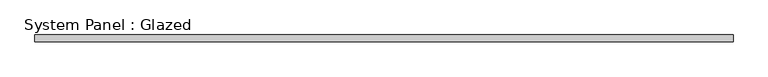
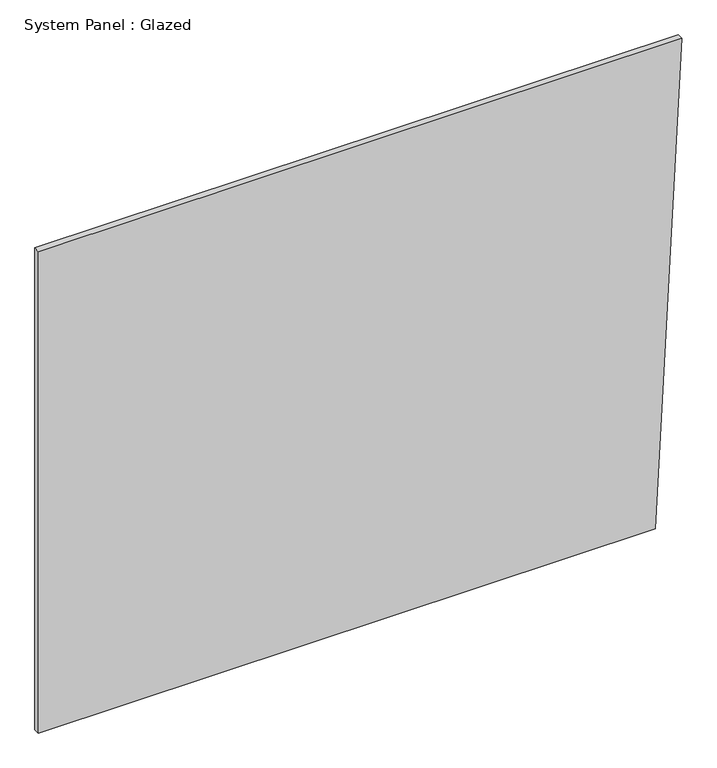
"""IFC4 building model written with IfcOpenShell, lengths in millimetres: plate geometry, System Panel : Glazed."""

import ifcopenshell
import ifcopenshell.guid

model = None  # the IFC model being written
_history = None  # IfcOwnerHistory: only IFC2X3 demands one
_inside = {}  # id of a spatial element -> (the spatial element, [elements in it])
_under = {}  # id of a project, library or spatial element -> (it, [spatial elements below it])
_declared = {}  # id of a project -> (the project, [libraries it declares])
_typed = {}  # id of a type object -> (the type object, [elements of that type])
_made_of = {}  # id of a material, layer set ... -> (it, [elements and type objects made of it])


def new_model(schema):
    """Start an empty IFC model of exactly this schema.

    Asked for "IFC4X3", IfcOpenShell would pick the latest addendum, in which some entities
    have other attributes; the version numbers below select the first issue.
    IFC2X3 requires an IfcOwnerHistory on every rooted entity: one is made here for all.
    """
    global model, _history
    if schema == "IFC4X3":
        model = ifcopenshell.file(schema_version=(4, 3, 0, 0))
    else:
        model = ifcopenshell.file(schema=schema)
    _inside.clear()
    _under.clear()
    _declared.clear()
    _typed.clear()
    _made_of.clear()
    _history = None
    if model.schema == "IFC2X3":
        org = make("IfcOrganization", Name="unknown")
        user = make(
            "IfcPersonAndOrganization",
            ThePerson=make("IfcPerson", FamilyName="unknown"),
            TheOrganization=org,
        )
        app = make(
            "IfcApplication",
            ApplicationDeveloper=org,
            Version="unknown",
            ApplicationFullName="unknown",
            ApplicationIdentifier="unknown",
        )
        _history = make(
            "IfcOwnerHistory",
            OwningUser=user,
            OwningApplication=app,
            ChangeAction="ADDED",
            CreationDate=0,
        )
    return model


def make(cls, **values):
    """One entity of the class cls with the attributes given. An attribute that is None is left unset."""
    return model.create_entity(
        cls, **{name: value for name, value in values.items() if value is not None}
    )


def rooted(cls, **values):
    """An entity with a GlobalId (a new one), such as an element, a storey or a relation."""
    return make(cls, GlobalId=ifcopenshell.guid.new(), OwnerHistory=_history, **values)


def si_unit(unit_type, name, prefix=None):
    """IfcSIUnit, for example si_unit("LENGTHUNIT", "METRE", prefix="MILLI")."""
    return make("IfcSIUnit", UnitType=unit_type, Prefix=prefix, Name=name)


def assignment(units):
    """IfcUnitAssignment: the units of a project."""
    return None if units is None else make("IfcUnitAssignment", Units=units)


def point(xyz):
    """IfcCartesianPoint."""
    return None if xyz is None else make("IfcCartesianPoint", Coordinates=xyz)


def direction(xyz):
    """IfcDirection."""
    return None if xyz is None else make("IfcDirection", DirectionRatios=xyz)


def frame(location, z_axis=None, x_axis=None):
    """IfcAxis2Placement3D, a coordinate frame: its origin and axes. An axis left out is left unset."""
    return make(
        "IfcAxis2Placement3D",
        Location=point(location),
        Axis=direction(z_axis),
        RefDirection=direction(x_axis),
    )


def origin():
    """The frame at (0, 0, 0) with its axes left unset."""
    return frame((0.0, 0.0, 0.0))


def place(relative_to, where):
    """IfcLocalPlacement: puts the frame where relative to a parent placement (None: the world)."""
    return make(
        "IfcLocalPlacement", PlacementRelTo=relative_to, RelativePlacement=where
    )


def context(
    kind, dimensions, precision=None, world=None, true_north=None, identifier=None
):
    """IfcGeometricRepresentationContext, for example the 3D "Model" context."""
    return make(
        "IfcGeometricRepresentationContext",
        ContextIdentifier=identifier,
        ContextType=kind,
        CoordinateSpaceDimension=dimensions,
        Precision=precision,
        WorldCoordinateSystem=world,
        TrueNorth=true_north,
    )


def project(units=None, contexts=None):
    """IfcProject with its units and contexts."""
    return rooted(
        "IfcProject",
        Name="project",
        RepresentationContexts=contexts,
        UnitsInContext=assignment(units),
    )


def spatial(cls, under=None, at=None, **own):
    """A site, building, storey or space (cls), placed at a placement, below another one or the project."""
    s = rooted(cls, ObjectPlacement=at, **own)
    if under is not None:
        _under.setdefault(under.id(), (under, []))[1].append(s)
    return s


def polyline(points):
    """IfcPolyline through the points."""
    return make("IfcPolyline", Points=[point(p) for p in points])


def outline(outer, holes=None, kind="AREA"):
    """IfcArbitraryClosedProfileDef: a profile drawn as a closed curve; with holes, ...WithVoids."""
    if holes is None:
        return make("IfcArbitraryClosedProfileDef", ProfileType=kind, OuterCurve=outer)
    return make(
        "IfcArbitraryProfileDefWithVoids",
        ProfileType=kind,
        OuterCurve=outer,
        InnerCurves=holes,
    )


def extrude(swept, where, along, depth):
    """IfcExtrudedAreaSolid: the profile swept, set in the frame where, extruded along a direction by depth."""
    return make(
        "IfcExtrudedAreaSolid",
        SweptArea=swept,
        Position=where,
        ExtrudedDirection=direction(along),
        Depth=depth,
    )


def shape(context_of_items, identifier, shape_type, items):
    """IfcShapeRepresentation: the items that make up one representation, for example the "Body"."""
    return make(
        "IfcShapeRepresentation",
        ContextOfItems=context_of_items,
        RepresentationIdentifier=identifier,
        RepresentationType=shape_type,
        Items=items,
    )


def source(mapping_origin, context_of_items, identifier, shape_type, items):
    """IfcRepresentationMap: a shape defined once, which mapped items show again and again."""
    return make(
        "IfcRepresentationMap",
        MappingOrigin=mapping_origin,
        MappedRepresentation=shape(context_of_items, identifier, shape_type, items),
    )


def transform(
    local_origin,
    x_axis=None,
    y_axis=None,
    z_axis=None,
    scale=None,
    scale2=None,
    scale3=None,
    uniform=True,
):
    """IfcCartesianTransformationOperator3D, or its non-uniform kind. x_axis, y_axis, z_axis: its Axis1, 2, 3."""
    if uniform:
        return make(
            "IfcCartesianTransformationOperator3D",
            Axis1=direction(x_axis),
            Axis2=direction(y_axis),
            LocalOrigin=point(local_origin),
            Scale=scale,
            Axis3=direction(z_axis),
        )
    return make(
        "IfcCartesianTransformationOperator3DnonUniform",
        Axis1=direction(x_axis),
        Axis2=direction(y_axis),
        LocalOrigin=point(local_origin),
        Scale=scale,
        Axis3=direction(z_axis),
        Scale2=scale2,
        Scale3=scale3,
    )


def mapped(mapping_source, mapping_target):
    """IfcMappedItem: shows the shape of a source again, moved by a transform."""
    return make(
        "IfcMappedItem", MappingSource=mapping_source, MappingTarget=mapping_target
    )


def made_of(thing, what):
    """Note that an element or type object is made of a material, layer set ...; save() writes the relation."""
    if what is not None:
        _made_of.setdefault(what.id(), (what, []))[1].append(thing)
    return thing


def element(
    cls,
    number,
    at=None,
    inside=None,
    cuts=None,
    type_object=None,
    material=None,
    context=None,
    identifier="Body",
    shape_type=None,
    held_by="IfcProductDefinitionShape",
    body=None,
    shapes=None,
    **own,
):
    """One element of the class cls, such as IfcWall. Its Tag is "e" and its number.

    at: its placement. inside: the storey or other place that contains it. cuts: it is an
    opening in that element (IfcRelVoidsElement). A single representation is given by context,
    identifier, shape_type and body (its items); several are given by shapes. held_by: the class
    of the entity that holds the representations. save() writes the other relations.
    """
    e = rooted(cls, Tag="e%d" % number, ObjectPlacement=at, **own)
    if body is not None:
        shapes = [shape(context, identifier, shape_type, body)]
    if shapes is not None:
        e.Representation = make(held_by, Representations=shapes)
    if inside is not None:
        _inside.setdefault(inside.id(), (inside, []))[1].append(e)
    if cuts is not None:
        rooted(
            "IfcRelVoidsElement", RelatingBuildingElement=cuts, RelatedOpeningElement=e
        )
    if type_object is not None:
        _typed.setdefault(type_object.id(), (type_object, []))[1].append(e)
    return made_of(e, material)


def aggregate(whole, parts):
    """IfcRelAggregates: a whole, such as a stair, and the parts it consists of."""
    return rooted("IfcRelAggregates", RelatingObject=whole, RelatedObjects=parts)


def save(model, path):
    """Write the relations noted so far, then the file.

    IfcRelAggregates (storeys below a building ...), IfcRelContainedInSpatialStructure (elements
    in a storey), IfcRelDefinesByType, IfcRelAssociatesMaterial and IfcRelDeclares: one each for
    every whole, place, type object, material and project.
    """
    for whole, parts in _under.values():
        aggregate(whole, parts)
    for where, things in _inside.values():
        rooted(
            "IfcRelContainedInSpatialStructure",
            RelatedElements=things,
            RelatingStructure=where,
        )
    for kind, things in _typed.values():
        rooted("IfcRelDefinesByType", RelatedObjects=things, RelatingType=kind)
    for what, things in _made_of.values():
        rooted("IfcRelAssociatesMaterial", RelatedObjects=things, RelatingMaterial=what)
    for by, libraries in _declared.values():
        rooted("IfcRelDeclares", RelatingContext=by, RelatedDefinitions=libraries)
    model.write(path)


def system_panel_glazed_f6a0a944(model_context):
    return source(origin(), model_context, "Body", "SweptSolid", [
        extrude(outline(polyline([(0.0, -1317.8741594), (0.0, 1208.7338763), (2085.3785982, 1317.8741594), (2085.3785982, -1317.8741594), (0.0, -1317.8741594)])), frame((0.0, -44.45, 0.0), z_axis=(0.0, 1.0, 0.0), x_axis=(0.0, 0.0, 1.0)), (0.0, 0.0, 1.0), 25.4),
    ])


if __name__ == "__main__":
    model = new_model("IFC4")
    model_context = context("Model", 3, world=origin())
    ifc_project = project(units=[si_unit("LENGTHUNIT", "METRE", prefix="MILLI")], contexts=[model_context])
    site = spatial("IfcSite", under=ifc_project)
    building = spatial("IfcBuilding", under=site)
    placement = place(None, origin())
    system_panel_glazed_shape = system_panel_glazed_f6a0a944(model_context)
    element("IfcPlate", 1, ObjectType="System Panel : Glazed", at=placement, inside=building, context=model_context, shape_type="MappedRepresentation", body=[
        mapped(system_panel_glazed_shape, transform((0.0, 0.0, 0.0), x_axis=(1.0, 0.0, 0.0), y_axis=(0.0, 1.0, 0.0), z_axis=(0.0, 0.0, 1.0))),
    ])
    save(model, "model.ifc")

# Revit data of these elements
# Type "System Panel : Glazed"
#   Construction Type Id = "GSP4R"
#   Analytic Construction = "1/8 in Pilkington single glazing"
#   Visual Light Transmittance = 0.9
#   Solar Heat Gain Coefficient = 0.86
#   Heat Transfer Coefficient (U) = 1.18115 BTU/(h·ft²·°F)
#   Define Thermal Properties by = 1
# Element 1 (IfcPlate, "System Panel : Glazed")
#   Materials on its faces: "Glass"
# Materials
#   "Glass": class "Glass", colour RGB 0 128 192, transparency 0.75, Description = "Soda Lime Glass", Cost = 0
